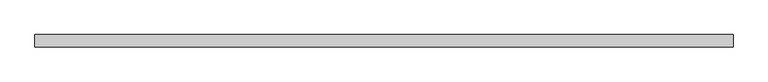
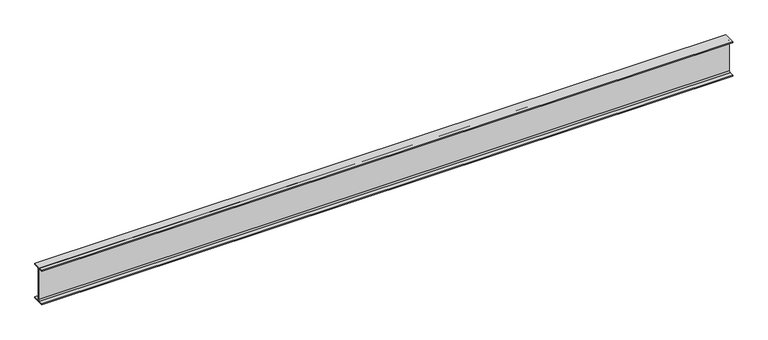
"""IFC4 building model written with IfcOpenShell, lengths in millimetres: beam geometry, Steel Framing_H_KS : H_SB_AR_S02_H-600x200x11x17_SRG2."""

import ifcopenshell
import ifcopenshell.guid

model = None  # the IFC model being written
_history = None  # IfcOwnerHistory: only IFC2X3 demands one
_inside = {}  # id of a spatial element -> (the spatial element, [elements in it])
_under = {}  # id of a project, library or spatial element -> (it, [spatial elements below it])
_declared = {}  # id of a project -> (the project, [libraries it declares])
_typed = {}  # id of a type object -> (the type object, [elements of that type])
_made_of = {}  # id of a material, layer set ... -> (it, [elements and type objects made of it])


def new_model(schema):
    """Start an empty IFC model of exactly this schema.

    Asked for "IFC4X3", IfcOpenShell would pick the latest addendum, in which some entities
    have other attributes; the version numbers below select the first issue.
    IFC2X3 requires an IfcOwnerHistory on every rooted entity: one is made here for all.
    """
    global model, _history
    if schema == "IFC4X3":
        model = ifcopenshell.file(schema_version=(4, 3, 0, 0))
    else:
        model = ifcopenshell.file(schema=schema)
    _inside.clear()
    _under.clear()
    _declared.clear()
    _typed.clear()
    _made_of.clear()
    _history = None
    if model.schema == "IFC2X3":
        org = make("IfcOrganization", Name="unknown")
        user = make(
            "IfcPersonAndOrganization",
            ThePerson=make("IfcPerson", FamilyName="unknown"),
            TheOrganization=org,
        )
        app = make(
            "IfcApplication",
            ApplicationDeveloper=org,
            Version="unknown",
            ApplicationFullName="unknown",
            ApplicationIdentifier="unknown",
        )
        _history = make(
            "IfcOwnerHistory",
            OwningUser=user,
            OwningApplication=app,
            ChangeAction="ADDED",
            CreationDate=0,
        )
    return model


def make(cls, **values):
    """One entity of the class cls with the attributes given. An attribute that is None is left unset."""
    return model.create_entity(
        cls, **{name: value for name, value in values.items() if value is not None}
    )


def rooted(cls, **values):
    """An entity with a GlobalId (a new one), such as an element, a storey or a relation."""
    return make(cls, GlobalId=ifcopenshell.guid.new(), OwnerHistory=_history, **values)


def si_unit(unit_type, name, prefix=None):
    """IfcSIUnit, for example si_unit("LENGTHUNIT", "METRE", prefix="MILLI")."""
    return make("IfcSIUnit", UnitType=unit_type, Prefix=prefix, Name=name)


def assignment(units):
    """IfcUnitAssignment: the units of a project."""
    return None if units is None else make("IfcUnitAssignment", Units=units)


def point(xyz):
    """IfcCartesianPoint."""
    return None if xyz is None else make("IfcCartesianPoint", Coordinates=xyz)


def direction(xyz):
    """IfcDirection."""
    return None if xyz is None else make("IfcDirection", DirectionRatios=xyz)


def frame(location, z_axis=None, x_axis=None):
    """IfcAxis2Placement3D, a coordinate frame: its origin and axes. An axis left out is left unset."""
    return make(
        "IfcAxis2Placement3D",
        Location=point(location),
        Axis=direction(z_axis),
        RefDirection=direction(x_axis),
    )


def frame_2d(location, x_axis=None):
    """IfcAxis2Placement2D, a coordinate frame in the plane: its origin and x axis."""
    return make(
        "IfcAxis2Placement2D", Location=point(location), RefDirection=direction(x_axis)
    )


def origin():
    """The frame at (0, 0, 0) with its axes left unset."""
    return frame((0.0, 0.0, 0.0))


def place(relative_to, where):
    """IfcLocalPlacement: puts the frame where relative to a parent placement (None: the world)."""
    return make(
        "IfcLocalPlacement", PlacementRelTo=relative_to, RelativePlacement=where
    )


def context(
    kind, dimensions, precision=None, world=None, true_north=None, identifier=None
):
    """IfcGeometricRepresentationContext, for example the 3D "Model" context."""
    return make(
        "IfcGeometricRepresentationContext",
        ContextIdentifier=identifier,
        ContextType=kind,
        CoordinateSpaceDimension=dimensions,
        Precision=precision,
        WorldCoordinateSystem=world,
        TrueNorth=true_north,
    )


def project(units=None, contexts=None):
    """IfcProject with its units and contexts."""
    return rooted(
        "IfcProject",
        Name="project",
        RepresentationContexts=contexts,
        UnitsInContext=assignment(units),
    )


def spatial(cls, under=None, at=None, **own):
    """A site, building, storey or space (cls), placed at a placement, below another one or the project."""
    s = rooted(cls, ObjectPlacement=at, **own)
    if under is not None:
        _under.setdefault(under.id(), (under, []))[1].append(s)
    return s


def polyline(points):
    """IfcPolyline through the points."""
    return make("IfcPolyline", Points=[point(p) for p in points])


def circle_curve(where, radius):
    """IfcCircle in the frame where."""
    return make("IfcCircle", Position=where, Radius=radius)


def trimmed(basis, trim1, trim2, sense, master):
    """IfcTrimmedCurve: the piece of a basis curve between two trims."""
    return make(
        "IfcTrimmedCurve",
        BasisCurve=basis,
        Trim1=trim1,
        Trim2=trim2,
        SenseAgreement=sense,
        MasterRepresentation=master,
    )


def segment(curve, same_sense, transition):
    """IfcCompositeCurveSegment."""
    return make(
        "IfcCompositeCurveSegment",
        Transition=transition,
        SameSense=same_sense,
        ParentCurve=curve,
    )


def composite_curve(segments, self_intersect=None):
    """IfcCompositeCurve: segments joined end to end."""
    return make("IfcCompositeCurve", Segments=segments, SelfIntersect=self_intersect)


def outline(outer, holes=None, kind="AREA"):
    """IfcArbitraryClosedProfileDef: a profile drawn as a closed curve; with holes, ...WithVoids."""
    if holes is None:
        return make("IfcArbitraryClosedProfileDef", ProfileType=kind, OuterCurve=outer)
    return make(
        "IfcArbitraryProfileDefWithVoids",
        ProfileType=kind,
        OuterCurve=outer,
        InnerCurves=holes,
    )


def extrude(swept, where, along, depth):
    """IfcExtrudedAreaSolid: the profile swept, set in the frame where, extruded along a direction by depth."""
    return make(
        "IfcExtrudedAreaSolid",
        SweptArea=swept,
        Position=where,
        ExtrudedDirection=direction(along),
        Depth=depth,
    )


def shape(context_of_items, identifier, shape_type, items):
    """IfcShapeRepresentation: the items that make up one representation, for example the "Body"."""
    return make(
        "IfcShapeRepresentation",
        ContextOfItems=context_of_items,
        RepresentationIdentifier=identifier,
        RepresentationType=shape_type,
        Items=items,
    )


def source(mapping_origin, context_of_items, identifier, shape_type, items):
    """IfcRepresentationMap: a shape defined once, which mapped items show again and again."""
    return make(
        "IfcRepresentationMap",
        MappingOrigin=mapping_origin,
        MappedRepresentation=shape(context_of_items, identifier, shape_type, items),
    )


def transform(
    local_origin,
    x_axis=None,
    y_axis=None,
    z_axis=None,
    scale=None,
    scale2=None,
    scale3=None,
    uniform=True,
):
    """IfcCartesianTransformationOperator3D, or its non-uniform kind. x_axis, y_axis, z_axis: its Axis1, 2, 3."""
    if uniform:
        return make(
            "IfcCartesianTransformationOperator3D",
            Axis1=direction(x_axis),
            Axis2=direction(y_axis),
            LocalOrigin=point(local_origin),
            Scale=scale,
            Axis3=direction(z_axis),
        )
    return make(
        "IfcCartesianTransformationOperator3DnonUniform",
        Axis1=direction(x_axis),
        Axis2=direction(y_axis),
        LocalOrigin=point(local_origin),
        Scale=scale,
        Axis3=direction(z_axis),
        Scale2=scale2,
        Scale3=scale3,
    )


def mapped(mapping_source, mapping_target):
    """IfcMappedItem: shows the shape of a source again, moved by a transform."""
    return make(
        "IfcMappedItem", MappingSource=mapping_source, MappingTarget=mapping_target
    )


def made_of(thing, what):
    """Note that an element or type object is made of a material, layer set ...; save() writes the relation."""
    if what is not None:
        _made_of.setdefault(what.id(), (what, []))[1].append(thing)
    return thing


def element(
    cls,
    number,
    at=None,
    inside=None,
    cuts=None,
    type_object=None,
    material=None,
    context=None,
    identifier="Body",
    shape_type=None,
    held_by="IfcProductDefinitionShape",
    body=None,
    shapes=None,
    **own,
):
    """One element of the class cls, such as IfcWall. Its Tag is "e" and its number.

    at: its placement. inside: the storey or other place that contains it. cuts: it is an
    opening in that element (IfcRelVoidsElement). A single representation is given by context,
    identifier, shape_type and body (its items); several are given by shapes. held_by: the class
    of the entity that holds the representations. save() writes the other relations.
    """
    e = rooted(cls, Tag="e%d" % number, ObjectPlacement=at, **own)
    if body is not None:
        shapes = [shape(context, identifier, shape_type, body)]
    if shapes is not None:
        e.Representation = make(held_by, Representations=shapes)
    if inside is not None:
        _inside.setdefault(inside.id(), (inside, []))[1].append(e)
    if cuts is not None:
        rooted(
            "IfcRelVoidsElement", RelatingBuildingElement=cuts, RelatedOpeningElement=e
        )
    if type_object is not None:
        _typed.setdefault(type_object.id(), (type_object, []))[1].append(e)
    return made_of(e, material)


def aggregate(whole, parts):
    """IfcRelAggregates: a whole, such as a stair, and the parts it consists of."""
    return rooted("IfcRelAggregates", RelatingObject=whole, RelatedObjects=parts)


def save(model, path):
    """Write the relations noted so far, then the file.

    IfcRelAggregates (storeys below a building ...), IfcRelContainedInSpatialStructure (elements
    in a storey), IfcRelDefinesByType, IfcRelAssociatesMaterial and IfcRelDeclares: one each for
    every whole, place, type object, material and project.
    """
    for whole, parts in _under.values():
        aggregate(whole, parts)
    for where, things in _inside.values():
        rooted(
            "IfcRelContainedInSpatialStructure",
            RelatedElements=things,
            RelatingStructure=where,
        )
    for kind, things in _typed.values():
        rooted("IfcRelDefinesByType", RelatedObjects=things, RelatingType=kind)
    for what, things in _made_of.values():
        rooted("IfcRelAssociatesMaterial", RelatedObjects=things, RelatingMaterial=what)
    for by, libraries in _declared.values():
        rooted("IfcRelDeclares", RelatingContext=by, RelatedDefinitions=libraries)
    model.write(path)


def beam_fedc1a72(model_context):
    return source(origin(), model_context, "Body", "SweptSolid", [
        extrude(outline(composite_curve([segment(polyline([(100.0, -283.0), (100.0, -300.0), (-100.0, -300.0), (-100.0, -283.0), (-27.5, -283.0)]), True, "CONTINUOUS"), segment(trimmed(circle_curve(frame_2d((-27.5, -261.0)), 22.0), [point((-27.5, -283.0))], [point((-5.5, -261.0))], True, "CARTESIAN"), True, "CONTINUOUS"), segment(polyline([(-5.5, -261.0), (-5.5, 261.0)]), True, "CONTINUOUS"), segment(trimmed(circle_curve(frame_2d((-27.5, 261.0)), 22.0), [point((-5.5, 261.0))], [point((-27.5, 283.0))], True, "CARTESIAN"), True, "CONTINUOUS"), segment(polyline([(-27.5, 283.0), (-100.0, 283.0), (-100.0, 300.0), (100.0, 300.0), (100.0, 283.0), (27.5, 283.0)]), True, "CONTINUOUS"), segment(trimmed(circle_curve(frame_2d((27.5, 261.0)), 22.0), [point((27.5, 283.0))], [point((5.5, 261.0))], True, "CARTESIAN"), True, "CONTINUOUS"), segment(polyline([(5.5, 261.0), (5.5, -261.0)]), True, "CONTINUOUS"), segment(trimmed(circle_curve(frame_2d((27.5, -261.0)), 22.0), [point((5.5, -261.0))], [point((27.5, -283.0))], True, "CARTESIAN"), True, "CONTINUOUS"), segment(polyline([(27.5, -283.0), (100.0, -283.0)]), True, "CONTINUOUS")], self_intersect=False)), frame((-5693.3, 0.0, 0.0), z_axis=(1.0, 0.0, 0.0), x_axis=(0.0, 1.0, 0.0)), (0.0, 0.0, 1.0), 11386.6),
    ])


if __name__ == "__main__":
    model = new_model("IFC4")
    model_context = context("Model", 3, world=origin())
    ifc_project = project(units=[si_unit("LENGTHUNIT", "METRE", prefix="MILLI")], contexts=[model_context])
    site = spatial("IfcSite", under=ifc_project)
    building = spatial("IfcBuilding", under=site)
    placement = place(None, origin())
    beam_shape = beam_fedc1a72(model_context)
    element("IfcBeam", 1, ObjectType="Steel Framing_H_KS : H_SB_AR_S02_H-600x200x11x17_SRG2", at=placement, inside=building, context=model_context, shape_type="MappedRepresentation", body=[
        mapped(beam_shape, transform((0.0, 0.0, 0.0), x_axis=(1.0, 0.0, 0.0), y_axis=(0.0, 1.0, 0.0), z_axis=(0.0, 0.0, 1.0))),
    ])
    save(model, "model.ifc")

# Revit data of these elements
# Type "Steel Framing_H_KS : H_SB_AR_S02_H-600x200x11x17_SRG2"
#   Type Comments = "MAIN"
#   Type Mark = "SRG2"
#   H_SectionID = "H-600x200x11x17"
#   H_Ratio for Additional Steel Plate = 0.2
#   Width = 20.0 cm
#   Web Thickness = 1.1 cm
#   Web Fillet = 2.2 cm
#   Warping Constant = 1930000.0 cm⁶
#   Torsional Moment of Inertia = 91.3724 cm⁴
#   Section Area = 134.4 cm²
#   Plastic Modulus weak axis = 361.0 cm³
#   Plastic Modulus strong axis = 2980.0 cm³
#   Perimeter = 1.94 m²/m
#   Nominal Weight = 106.00 kgf/m
#   Moment of Inertia weak axis = 2280.00 cm⁴
#   Moment of Inertia strong axis = 77600.00 cm⁴
#   Height = 60.0 cm
#   Flange Thickness = 1.7 cm
#   Elastic Modulus weak axis = 228.0 cm³
#   Elastic Modulus strong axis = 2590.0 cm³
#   Centroid Vertical = 30.0 cm
#   Centroid Horizontal = 10.0 cm
#   Bolt Spacing = 8.89 cm
#   Length [instance default] = 1500 mm
#   Structural Material [instance default] = Steel, 45-345
#   Section Name Key = ""
#   Assembly Code = ""
# Element 1 (IfcBeam, "Steel Framing_H_KS : H_SB_AR_S02_H-600x200x11x17_SRG2")
#   Materials on its faces: "Steel, 45-345"
# Materials
#   "Steel, 45-345": class "Metal", colour RGB 189 187 185, transparency 0, Description = "Steel 345 MPa", Cost = 0
